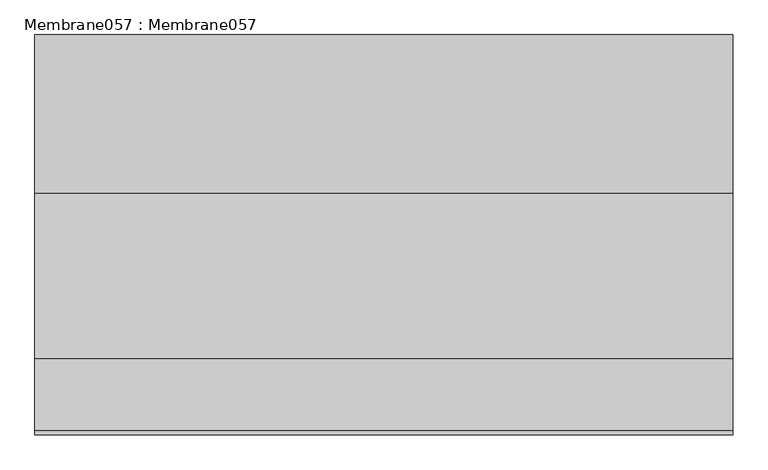
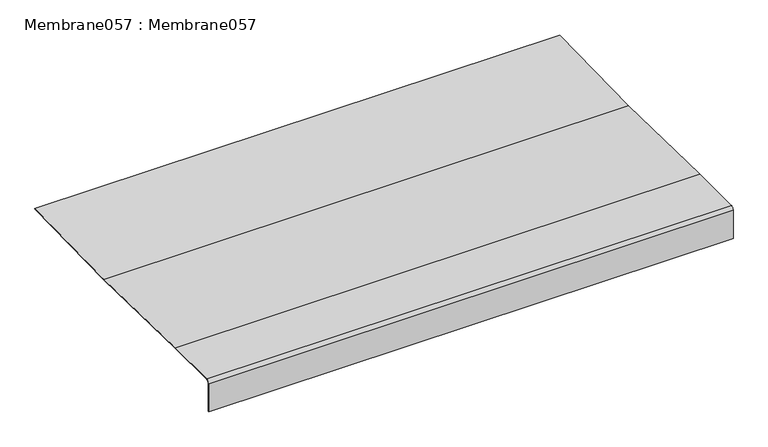
"""IFC4 building model written with IfcOpenShell, lengths in millimetres: proxy geometry, Membrane057 : Membrane057."""

import ifcopenshell
import ifcopenshell.guid

model = None  # the IFC model being written
_history = None  # IfcOwnerHistory: only IFC2X3 demands one
_inside = {}  # id of a spatial element -> (the spatial element, [elements in it])
_under = {}  # id of a project, library or spatial element -> (it, [spatial elements below it])
_declared = {}  # id of a project -> (the project, [libraries it declares])
_typed = {}  # id of a type object -> (the type object, [elements of that type])
_made_of = {}  # id of a material, layer set ... -> (it, [elements and type objects made of it])


def new_model(schema):
    """Start an empty IFC model of exactly this schema.

    Asked for "IFC4X3", IfcOpenShell would pick the latest addendum, in which some entities
    have other attributes; the version numbers below select the first issue.
    IFC2X3 requires an IfcOwnerHistory on every rooted entity: one is made here for all.
    """
    global model, _history
    if schema == "IFC4X3":
        model = ifcopenshell.file(schema_version=(4, 3, 0, 0))
    else:
        model = ifcopenshell.file(schema=schema)
    _inside.clear()
    _under.clear()
    _declared.clear()
    _typed.clear()
    _made_of.clear()
    _history = None
    if model.schema == "IFC2X3":
        org = make("IfcOrganization", Name="unknown")
        user = make(
            "IfcPersonAndOrganization",
            ThePerson=make("IfcPerson", FamilyName="unknown"),
            TheOrganization=org,
        )
        app = make(
            "IfcApplication",
            ApplicationDeveloper=org,
            Version="unknown",
            ApplicationFullName="unknown",
            ApplicationIdentifier="unknown",
        )
        _history = make(
            "IfcOwnerHistory",
            OwningUser=user,
            OwningApplication=app,
            ChangeAction="ADDED",
            CreationDate=0,
        )
    return model


def make(cls, **values):
    """One entity of the class cls with the attributes given. An attribute that is None is left unset."""
    return model.create_entity(
        cls, **{name: value for name, value in values.items() if value is not None}
    )


def rooted(cls, **values):
    """An entity with a GlobalId (a new one), such as an element, a storey or a relation."""
    return make(cls, GlobalId=ifcopenshell.guid.new(), OwnerHistory=_history, **values)


def si_unit(unit_type, name, prefix=None):
    """IfcSIUnit, for example si_unit("LENGTHUNIT", "METRE", prefix="MILLI")."""
    return make("IfcSIUnit", UnitType=unit_type, Prefix=prefix, Name=name)


def assignment(units):
    """IfcUnitAssignment: the units of a project."""
    return None if units is None else make("IfcUnitAssignment", Units=units)


def point(xyz):
    """IfcCartesianPoint."""
    return None if xyz is None else make("IfcCartesianPoint", Coordinates=xyz)


def direction(xyz):
    """IfcDirection."""
    return None if xyz is None else make("IfcDirection", DirectionRatios=xyz)


def frame(location, z_axis=None, x_axis=None):
    """IfcAxis2Placement3D, a coordinate frame: its origin and axes. An axis left out is left unset."""
    return make(
        "IfcAxis2Placement3D",
        Location=point(location),
        Axis=direction(z_axis),
        RefDirection=direction(x_axis),
    )


def frame_2d(location, x_axis=None):
    """IfcAxis2Placement2D, a coordinate frame in the plane: its origin and x axis."""
    return make(
        "IfcAxis2Placement2D", Location=point(location), RefDirection=direction(x_axis)
    )


def origin():
    """The frame at (0, 0, 0) with its axes left unset."""
    return frame((0.0, 0.0, 0.0))


def place(relative_to, where):
    """IfcLocalPlacement: puts the frame where relative to a parent placement (None: the world)."""
    return make(
        "IfcLocalPlacement", PlacementRelTo=relative_to, RelativePlacement=where
    )


def context(
    kind, dimensions, precision=None, world=None, true_north=None, identifier=None
):
    """IfcGeometricRepresentationContext, for example the 3D "Model" context."""
    return make(
        "IfcGeometricRepresentationContext",
        ContextIdentifier=identifier,
        ContextType=kind,
        CoordinateSpaceDimension=dimensions,
        Precision=precision,
        WorldCoordinateSystem=world,
        TrueNorth=true_north,
    )


def project(units=None, contexts=None):
    """IfcProject with its units and contexts."""
    return rooted(
        "IfcProject",
        Name="project",
        RepresentationContexts=contexts,
        UnitsInContext=assignment(units),
    )


def spatial(cls, under=None, at=None, **own):
    """A site, building, storey or space (cls), placed at a placement, below another one or the project."""
    s = rooted(cls, ObjectPlacement=at, **own)
    if under is not None:
        _under.setdefault(under.id(), (under, []))[1].append(s)
    return s


def polyline(points):
    """IfcPolyline through the points."""
    return make("IfcPolyline", Points=[point(p) for p in points])


def circle_curve(where, radius):
    """IfcCircle in the frame where."""
    return make("IfcCircle", Position=where, Radius=radius)


def trimmed(basis, trim1, trim2, sense, master):
    """IfcTrimmedCurve: the piece of a basis curve between two trims."""
    return make(
        "IfcTrimmedCurve",
        BasisCurve=basis,
        Trim1=trim1,
        Trim2=trim2,
        SenseAgreement=sense,
        MasterRepresentation=master,
    )


def segment(curve, same_sense, transition):
    """IfcCompositeCurveSegment."""
    return make(
        "IfcCompositeCurveSegment",
        Transition=transition,
        SameSense=same_sense,
        ParentCurve=curve,
    )


def composite_curve(segments, self_intersect=None):
    """IfcCompositeCurve: segments joined end to end."""
    return make("IfcCompositeCurve", Segments=segments, SelfIntersect=self_intersect)


def outline(outer, holes=None, kind="AREA"):
    """IfcArbitraryClosedProfileDef: a profile drawn as a closed curve; with holes, ...WithVoids."""
    if holes is None:
        return make("IfcArbitraryClosedProfileDef", ProfileType=kind, OuterCurve=outer)
    return make(
        "IfcArbitraryProfileDefWithVoids",
        ProfileType=kind,
        OuterCurve=outer,
        InnerCurves=holes,
    )


def extrude(swept, where, along, depth):
    """IfcExtrudedAreaSolid: the profile swept, set in the frame where, extruded along a direction by depth."""
    return make(
        "IfcExtrudedAreaSolid",
        SweptArea=swept,
        Position=where,
        ExtrudedDirection=direction(along),
        Depth=depth,
    )


def shape(context_of_items, identifier, shape_type, items):
    """IfcShapeRepresentation: the items that make up one representation, for example the "Body"."""
    return make(
        "IfcShapeRepresentation",
        ContextOfItems=context_of_items,
        RepresentationIdentifier=identifier,
        RepresentationType=shape_type,
        Items=items,
    )


def source(mapping_origin, context_of_items, identifier, shape_type, items):
    """IfcRepresentationMap: a shape defined once, which mapped items show again and again."""
    return make(
        "IfcRepresentationMap",
        MappingOrigin=mapping_origin,
        MappedRepresentation=shape(context_of_items, identifier, shape_type, items),
    )


def transform(
    local_origin,
    x_axis=None,
    y_axis=None,
    z_axis=None,
    scale=None,
    scale2=None,
    scale3=None,
    uniform=True,
):
    """IfcCartesianTransformationOperator3D, or its non-uniform kind. x_axis, y_axis, z_axis: its Axis1, 2, 3."""
    if uniform:
        return make(
            "IfcCartesianTransformationOperator3D",
            Axis1=direction(x_axis),
            Axis2=direction(y_axis),
            LocalOrigin=point(local_origin),
            Scale=scale,
            Axis3=direction(z_axis),
        )
    return make(
        "IfcCartesianTransformationOperator3DnonUniform",
        Axis1=direction(x_axis),
        Axis2=direction(y_axis),
        LocalOrigin=point(local_origin),
        Scale=scale,
        Axis3=direction(z_axis),
        Scale2=scale2,
        Scale3=scale3,
    )


def mapped(mapping_source, mapping_target):
    """IfcMappedItem: shows the shape of a source again, moved by a transform."""
    return make(
        "IfcMappedItem", MappingSource=mapping_source, MappingTarget=mapping_target
    )


def made_of(thing, what):
    """Note that an element or type object is made of a material, layer set ...; save() writes the relation."""
    if what is not None:
        _made_of.setdefault(what.id(), (what, []))[1].append(thing)
    return thing


def element(
    cls,
    number,
    at=None,
    inside=None,
    cuts=None,
    type_object=None,
    material=None,
    context=None,
    identifier="Body",
    shape_type=None,
    held_by="IfcProductDefinitionShape",
    body=None,
    shapes=None,
    **own,
):
    """One element of the class cls, such as IfcWall. Its Tag is "e" and its number.

    at: its placement. inside: the storey or other place that contains it. cuts: it is an
    opening in that element (IfcRelVoidsElement). A single representation is given by context,
    identifier, shape_type and body (its items); several are given by shapes. held_by: the class
    of the entity that holds the representations. save() writes the other relations.
    """
    e = rooted(cls, Tag="e%d" % number, ObjectPlacement=at, **own)
    if body is not None:
        shapes = [shape(context, identifier, shape_type, body)]
    if shapes is not None:
        e.Representation = make(held_by, Representations=shapes)
    if inside is not None:
        _inside.setdefault(inside.id(), (inside, []))[1].append(e)
    if cuts is not None:
        rooted(
            "IfcRelVoidsElement", RelatingBuildingElement=cuts, RelatedOpeningElement=e
        )
    if type_object is not None:
        _typed.setdefault(type_object.id(), (type_object, []))[1].append(e)
    return made_of(e, material)


def aggregate(whole, parts):
    """IfcRelAggregates: a whole, such as a stair, and the parts it consists of."""
    return rooted("IfcRelAggregates", RelatingObject=whole, RelatedObjects=parts)


def save(model, path):
    """Write the relations noted so far, then the file.

    IfcRelAggregates (storeys below a building ...), IfcRelContainedInSpatialStructure (elements
    in a storey), IfcRelDefinesByType, IfcRelAssociatesMaterial and IfcRelDeclares: one each for
    every whole, place, type object, material and project.
    """
    for whole, parts in _under.values():
        aggregate(whole, parts)
    for where, things in _inside.values():
        rooted(
            "IfcRelContainedInSpatialStructure",
            RelatedElements=things,
            RelatingStructure=where,
        )
    for kind, things in _typed.values():
        rooted("IfcRelDefinesByType", RelatedObjects=things, RelatingType=kind)
    for what, things in _made_of.values():
        rooted("IfcRelAssociatesMaterial", RelatedObjects=things, RelatingMaterial=what)
    for by, libraries in _declared.values():
        rooted("IfcRelDeclares", RelatingContext=by, RelatedDefinitions=libraries)
    model.write(path)


def membrane057_membrane057_1e3ff11b(model_context):
    return source(origin(), model_context, "Body", "SweptSolid", [
        extrude(outline(composite_curve([segment(polyline([(-5567.4209762, 40106.229319), (-5569.4209762, 40106.229319), (-5569.4209762, 40219.8534812)]), True, "CONTINUOUS"), segment(trimmed(circle_curve(frame_2d((-5557.4209762, 40219.8534812)), 12.0), [point((-5569.4209762, 40219.8534812))], [point((-5557.4209762, 40231.8534812))], False, "CARTESIAN"), True, "CONTINUOUS"), segment(polyline([(-5557.4209762, 40231.8534812), (-5350.1524727, 40231.8534812), (-4876.5591046, 40221.0182087), (-4423.1183678, 40230.8349368), (-4423.0750791, 40228.8354053), (-4876.5603336, 40219.0177134), (-5350.1753483, 40229.8534812), (-5557.4209762, 40229.8534812)]), True, "CONTINUOUS"), segment(trimmed(circle_curve(frame_2d((-5557.4209762, 40219.8534812)), 10.0), [point((-5557.4209762, 40229.8534812))], [point((-5567.4209762, 40219.8534812))], True, "CARTESIAN"), True, "CONTINUOUS"), segment(polyline([(-5567.4209762, 40219.8534812), (-5567.4209762, 40106.229319)]), True, "CONTINUOUS")], self_intersect=False)), frame((12383.0178845, 0.0, 0.0), z_axis=(1.0, 0.0, 0.0), x_axis=(0.0, 1.0, 0.0)), (0.0, 0.0, 1.0), 2000.0),
    ])


if __name__ == "__main__":
    model = new_model("IFC4")
    model_context = context("Model", 3, world=origin())
    ifc_project = project(units=[si_unit("LENGTHUNIT", "METRE", prefix="MILLI")], contexts=[model_context])
    site = spatial("IfcSite", under=ifc_project)
    building = spatial("IfcBuilding", under=site)
    placement = place(None, origin())
    membrane057_membrane057_shape = membrane057_membrane057_1e3ff11b(model_context)
    element("IfcBuildingElementProxy", 1, Name="Membrane057 : Membrane057", ObjectType="Membrane057 : Membrane057", at=placement, inside=building, context=model_context, shape_type="MappedRepresentation", body=[
        mapped(membrane057_membrane057_shape, transform((0.0, 0.0, 0.0), x_axis=(1.0, 0.0, 0.0), y_axis=(0.0, 1.0, 0.0), z_axis=(0.0, 0.0, 1.0))),
    ])
    save(model, "model.ifc")

# Revit data of these elements
# Type "Membrane057 : Membrane057"
#   NameOverride = "Membrane057"
# Element 1 (IfcBuildingElementProxy, "Membrane057 : Membrane057")
#   Materials on its faces: "THREE PLY BUILT UP ROOF MEMBRANE"
# Materials
#   "THREE PLY BUILT UP ROOF MEMBRANE": class "Unassigned", colour RGB 63 63 63, transparency 0
